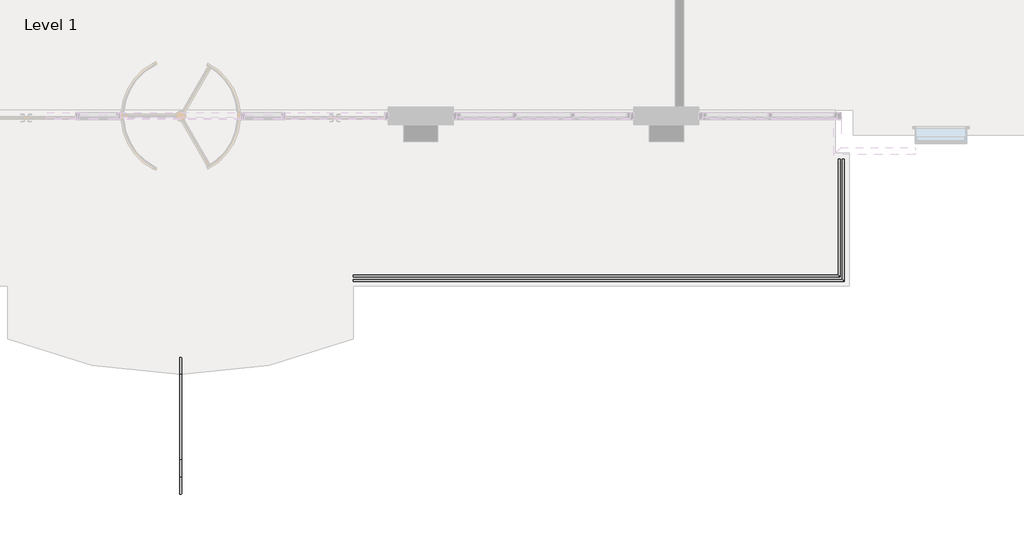
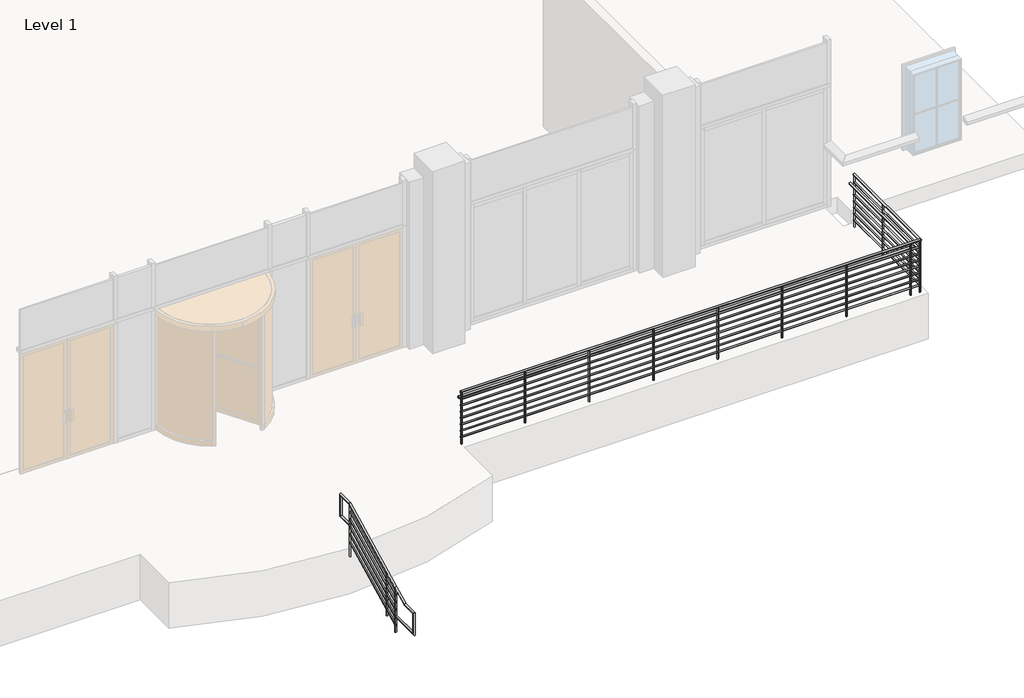
# One storey, part 4 of 6: 2 railings.
"""IFC4 building model written with IfcOpenShell, lengths in millimetres."""

from ifc_helpers import new_model, si_unit, point, frame, frame_2d, origin, origin_with_axes, place, context, project, spatial, circle_curve, ellipse_curve, trimmed, segment, composite_curve, outline, extrude, element, save
from ifc_brep_helpers import plane_surface, cylinder_surface, advanced_brep

model = new_model("IFC4")

# Units and contexts
model_context = context("Model", 3, world=origin())
ifc_project = project(units=[si_unit("LENGTHUNIT", "METRE", prefix="MILLI")], contexts=[model_context])

# Site, building, storey
site = spatial("IfcSite", under=ifc_project)
building = spatial("IfcBuilding", under=site)
storey = spatial("IfcBuildingStorey", under=building, Name="Level 1", Elevation=0.0)

# Railings
placement = place(None, origin())
element("IfcRailing", 1, ObjectType="Handrail – Pipe – Bottom &Top Extension", at=placement, inside=storey, context=model_context, shape_type="AdvancedBrep", body=[
    advanced_brep(
    [(-1146.7622732, -15471.359437, -438.15), (-1184.8622732, -15471.359437, -438.15), (-1146.7622732, -16062.2278525, -438.15), (-1184.8622732, -16062.2278525, -438.15), (-1146.7622732, -16062.2278525, -19.05), (-1184.8622732, -16062.2278525, -19.05), (-1146.7622732, -15771.9807575, -19.05), (-1184.8622732, -15771.9807575, -19.05), (-1146.7622732, -15463.1584335, 135.361162), (-1184.8622732, -15463.1584335, 135.361162), (-1146.7622732, -13943.1807575, 895.35), (-1184.8622732, -13943.1807575, 895.35), (-1146.7622732, -13661.9278525, 895.35), (-1184.8622732, -13661.9278525, 895.35), (-1146.7622732, -13661.9278525, 476.25), (-1184.8622732, -13661.9278525, 476.25), (-1146.7622732, -13947.996268, 476.25), (-1184.8622732, -13947.996268, 476.25)],
    [
        (0, 1, circle_curve(frame((-1165.8122732, -15471.359437, -438.15), z_axis=(0.0, 1.0, 0.0), x_axis=(-1.0, 0.0, 0.0)), 19.05)),
        (1, 0, circle_curve(frame((-1165.8122732, -15471.359437, -438.15), z_axis=(0.0, 1.0, 0.0), x_axis=(-1.0, 0.0, 0.0)), 19.05)),
        (0, 2),
        (2, 3, ellipse_curve(frame((-1165.8122732, -16062.2278525, -438.15), z_axis=(0.0, 0.7071067811865475, -0.7071067811865475), x_axis=(0.0, 0.7071067811865476, 0.7071067811865474)), 26.9407684, 19.05)),
        (3, 1),
        (3, 2, ellipse_curve(frame((-1165.8122732, -16062.2278525, -438.15), z_axis=(0.0, 0.7071067811865475, -0.7071067811865475), x_axis=(0.0, 0.7071067811865476, 0.7071067811865474)), 26.9407684, 19.05)),
        (2, 4),
        (4, 5, ellipse_curve(frame((-1165.8122732, -16062.2278525, -19.05), z_axis=(0.0, -0.7071067811865475, -0.7071067811865475), x_axis=(0.0, 0.7071067811865474, -0.7071067811865476)), 26.9407684, 19.05)),
        (5, 3),
        (5, 4, ellipse_curve(frame((-1165.8122732, -16062.2278525, -19.05), z_axis=(0.0, -0.7071067811865475, -0.7071067811865475), x_axis=(0.0, 0.7071067811865474, -0.7071067811865476)), 26.9407684, 19.05)),
        (4, 6),
        (6, 7, ellipse_curve(frame((-1165.8122732, -15771.9807575, -19.05), z_axis=(0.0, -0.9732489894677302, -0.22975292054736124), x_axis=(0.0, -0.22975292054736096, 0.9732489894677302)), 19.573614, 19.05)),
        (7, 5),
        (7, 6, ellipse_curve(frame((-1165.8122732, -15771.9807575, -19.05), z_axis=(0.0, -0.9732489894677302, -0.22975292054736124), x_axis=(0.0, -0.22975292054736096, 0.9732489894677302)), 19.573614, 19.05)),
        (6, 8),
        (8, 9, circle_curve(frame((-1165.8122732, -15463.1584335, 135.361162), z_axis=(0.0, -0.8944271909999159, -0.44721359549995804), x_axis=(-1.0, 0.0, 0.0)), 19.05)),
        (9, 7),
        (9, 8, circle_curve(frame((-1165.8122732, -15463.1584335, 135.361162), z_axis=(0.0, -0.8944271909999159, -0.44721359549995804), x_axis=(-1.0, 0.0, 0.0)), 19.05)),
        (8, 10),
        (10, 11, ellipse_curve(frame((-1165.8122732, -13943.1807575, 895.35), z_axis=(0.0, -0.9732489894677302, -0.22975292054736132), x_axis=(0.0, 0.2297529205473615, -0.9732489894677301)), 19.573614, 19.05)),
        (11, 9),
        (11, 10, ellipse_curve(frame((-1165.8122732, -13943.1807575, 895.35), z_axis=(0.0, -0.9732489894677302, -0.22975292054736132), x_axis=(0.0, 0.2297529205473615, -0.9732489894677301)), 19.573614, 19.05)),
        (10, 12),
        (12, 13, ellipse_curve(frame((-1165.8122732, -13661.9278525, 895.35), z_axis=(0.0, -0.7071067811865476, 0.7071067811865474), x_axis=(0.0, -0.7071067811865475, -0.7071067811865475)), 26.9407684, 19.05)),
        (13, 11),
        (13, 12, ellipse_curve(frame((-1165.8122732, -13661.9278525, 895.35), z_axis=(0.0, -0.7071067811865476, 0.7071067811865474), x_axis=(0.0, -0.7071067811865475, -0.7071067811865475)), 26.9407684, 19.05)),
        (12, 14),
        (14, 15, ellipse_curve(frame((-1165.8122732, -13661.9278525, 476.25), z_axis=(0.0, 0.7071067811865474, 0.7071067811865476), x_axis=(0.0, -0.7071067811865475, 0.7071067811865475)), 26.9407684, 19.05)),
        (15, 13),
        (15, 14, ellipse_curve(frame((-1165.8122732, -13661.9278525, 476.25), z_axis=(0.0, 0.7071067811865474, 0.7071067811865476), x_axis=(0.0, -0.7071067811865475, 0.7071067811865475)), 26.9407684, 19.05)),
        (16, 17, circle_curve(frame((-1165.8122732, -13947.996268, 476.25), z_axis=(0.0, -1.0, 0.0), x_axis=(-1.0, 0.0, 0.0)), 19.05)),
        (17, 16, circle_curve(frame((-1165.8122732, -13947.996268, 476.25), z_axis=(0.0, -1.0, 0.0), x_axis=(-1.0, 0.0, 0.0)), 19.05)),
        (14, 16),
        (17, 15),
    ],
    [
        plane_surface(frame((-1165.8122732, -15471.359437, -457.2), z_axis=(0.0, 1.0, 0.0), x_axis=(0.0, 0.0, -1.0))),
        cylinder_surface(frame((-1165.8122732, -15471.359437, -438.15), z_axis=(0.0, 1.0, 0.0), x_axis=(-1.0, 0.0, 0.0)), 19.05),
        cylinder_surface(frame((-1165.8122732, -16062.2278525, -457.2), z_axis=(0.0, 0.0, -1.0), x_axis=(-1.0, 0.0, 0.0)), 19.05),
        cylinder_surface(frame((-1165.8122732, -16081.2778525, -19.05), z_axis=(0.0, -1.0, 0.0), x_axis=(-1.0, 0.0, 0.0)), 19.05),
        cylinder_surface(frame((-1165.8122732, -15767.9584335, -17.038838), z_axis=(0.0, -0.8944271909999159, -0.44721359549995804), x_axis=(-1.0, 0.0, 0.0)), 19.05),
        cylinder_surface(frame((-1165.8122732, -15463.1584335, 135.361162), z_axis=(0.0, -0.8944271909999159, -0.44721359549995804), x_axis=(-1.0, 0.0, 0.0)), 19.05),
        cylinder_surface(frame((-1165.8122732, -13947.6778525, 895.35), z_axis=(0.0, -1.0, 0.0), x_axis=(-1.0, 0.0, 0.0)), 19.05),
        cylinder_surface(frame((-1165.8122732, -13661.9278525, 914.4), z_axis=(0.0, 0.0, 1.0), x_axis=(-1.0, 0.0, 0.0)), 19.05),
        plane_surface(frame((-1165.8122732, -13947.996268, 457.2), z_axis=(0.0, -1.0, 0.0), x_axis=(0.0, 0.0, -1.0))),
        cylinder_surface(frame((-1165.8122732, -13642.8778525, 476.25), z_axis=(0.0, 1.0, 0.0), x_axis=(-1.0, 0.0, 0.0)), 19.05),
    ],
    [
        (0, [[1, 2]]),
        (1, [[-1, 3, 4, 5]]),
        (1, [[-2, -5, 6, -3]]),
        (2, [[-4, 7, 8, 9]]),
        (2, [[-6, -9, 10, -7]]),
        (3, [[-8, 11, 12, 13]]),
        (3, [[-10, -13, 14, -11]]),
        (4, [[-12, 15, 16, 17]]),
        (4, [[-14, -17, 18, -15]]),
        (5, [[-16, 19, 20, 21]]),
        (5, [[-18, -21, 22, -19]]),
        (6, [[-20, 23, 24, 25]]),
        (6, [[-22, -25, 26, -23]]),
        (7, [[-24, 27, 28, 29]]),
        (7, [[-26, -29, 30, -27]]),
        (8, [[31, 32]]),
        (9, [[-28, 33, -32, 34]]),
        (9, [[-30, -34, -31, -33]]),
    ],
),
    advanced_brep(
    [(-1153.1122732, -13947.6778525, 747.8009683), (-1178.5122732, -13947.6778525, 747.8009683), (-1153.1122732, -15471.6778525, -14.1990317), (-1178.5122732, -15471.6778525, -14.1990317)],
    [
        (0, 1, ellipse_curve(frame((-1165.8122732, -13947.6778525, 747.8009683), z_axis=(0.0, 1.0, 0.0), x_axis=(0.0, 0.0, 1.0)), 14.1990317, 12.7)),
        (1, 0, ellipse_curve(frame((-1165.8122732, -13947.6778525, 747.8009683), z_axis=(0.0, 1.0, 0.0), x_axis=(0.0, 0.0, 1.0)), 14.1990317, 12.7)),
        (2, 3, ellipse_curve(frame((-1165.8122732, -15471.6778525, -14.1990317), z_axis=(0.0, -1.0, 0.0), x_axis=(0.0, 0.0, 1.0)), 14.1990317, 12.7)),
        (3, 2, ellipse_curve(frame((-1165.8122732, -15471.6778525, -14.1990317), z_axis=(0.0, -1.0, 0.0), x_axis=(0.0, 0.0, 1.0)), 14.1990317, 12.7)),
        (0, 2),
        (3, 1),
    ],
    [
        plane_surface(frame((-1165.8122732, -13947.6778525, 762.0), z_axis=(0.0, 1.0, 0.0), x_axis=(0.0, 0.0, -1.0))),
        plane_surface(frame((-1165.8122732, -15471.6778525, 0.0), z_axis=(0.0, -1.0, 0.0), x_axis=(0.0, 0.0, -1.0))),
        cylinder_surface(frame((-1165.8122732, -13941.9982398, 750.6407747), z_axis=(0.0, 0.894427190999916, 0.447213595499958), x_axis=(-1.0, 0.0, 0.0)), 12.7),
    ],
    [
        (0, [[1, 2]]),
        (1, [[3, 4]]),
        (2, [[-1, 5, -4, 6]]),
        (2, [[-2, -6, -3, -5]]),
    ],
),
    advanced_brep(
    [(-1153.1122732, -13947.6778525, 595.4009683), (-1178.5122732, -13947.6778525, 595.4009683), (-1153.1122732, -15471.6778525, -166.5990317), (-1178.5122732, -15471.6778525, -166.5990317)],
    [
        (0, 1, ellipse_curve(frame((-1165.8122732, -13947.6778525, 595.4009683), z_axis=(0.0, 1.0, 0.0), x_axis=(0.0, 0.0, 1.0)), 14.1990317, 12.7)),
        (1, 0, ellipse_curve(frame((-1165.8122732, -13947.6778525, 595.4009683), z_axis=(0.0, 1.0, 0.0), x_axis=(0.0, 0.0, 1.0)), 14.1990317, 12.7)),
        (2, 3, ellipse_curve(frame((-1165.8122732, -15471.6778525, -166.5990317), z_axis=(0.0, -1.0, 0.0), x_axis=(0.0, 0.0, 1.0)), 14.1990317, 12.7)),
        (3, 2, ellipse_curve(frame((-1165.8122732, -15471.6778525, -166.5990317), z_axis=(0.0, -1.0, 0.0), x_axis=(0.0, 0.0, 1.0)), 14.1990317, 12.7)),
        (0, 2),
        (3, 1),
    ],
    [
        plane_surface(frame((-1165.8122732, -13947.6778525, 609.6), z_axis=(0.0, 1.0, 0.0), x_axis=(0.0, 0.0, -1.0))),
        plane_surface(frame((-1165.8122732, -15471.6778525, -152.4), z_axis=(0.0, -1.0, 0.0), x_axis=(0.0, 0.0, -1.0))),
        cylinder_surface(frame((-1165.8122732, -13941.9982398, 598.2407747), z_axis=(0.0, 0.894427190999916, 0.447213595499958), x_axis=(-1.0, 0.0, 0.0)), 12.7),
    ],
    [
        (0, [[1, 2]]),
        (1, [[3, 4]]),
        (2, [[-1, 5, -4, 6]]),
        (2, [[-2, -6, -3, -5]]),
    ],
),
    advanced_brep(
    [(-1153.1122732, -13947.6778525, 443.0009683), (-1178.5122732, -13947.6778525, 443.0009683), (-1153.1122732, -15471.6778525, -318.9990317), (-1178.5122732, -15471.6778525, -318.9990317)],
    [
        (0, 1, ellipse_curve(frame((-1165.8122732, -13947.6778525, 443.0009683), z_axis=(0.0, 1.0, 0.0), x_axis=(0.0, 0.0, 1.0)), 14.1990317, 12.7)),
        (1, 0, ellipse_curve(frame((-1165.8122732, -13947.6778525, 443.0009683), z_axis=(0.0, 1.0, 0.0), x_axis=(0.0, 0.0, 1.0)), 14.1990317, 12.7)),
        (2, 3, ellipse_curve(frame((-1165.8122732, -15471.6778525, -318.9990317), z_axis=(0.0, -1.0, 0.0), x_axis=(0.0, 0.0, 1.0)), 14.1990317, 12.7)),
        (3, 2, ellipse_curve(frame((-1165.8122732, -15471.6778525, -318.9990317), z_axis=(0.0, -1.0, 0.0), x_axis=(0.0, 0.0, 1.0)), 14.1990317, 12.7)),
        (0, 2),
        (3, 1),
    ],
    [
        plane_surface(frame((-1165.8122732, -13947.6778525, 457.2), z_axis=(0.0, 1.0, 0.0), x_axis=(0.0, 0.0, -1.0))),
        plane_surface(frame((-1165.8122732, -15471.6778525, -304.8), z_axis=(0.0, -1.0, 0.0), x_axis=(0.0, 0.0, -1.0))),
        cylinder_surface(frame((-1165.8122732, -13941.9982398, 445.8407747), z_axis=(0.0, 0.894427190999916, 0.447213595499958), x_axis=(-1.0, 0.0, 0.0)), 12.7),
    ],
    [
        (0, [[1, 2]]),
        (1, [[3, 4]]),
        (2, [[-1, 5, -4, 6]]),
        (2, [[-2, -6, -3, -5]]),
    ],
),
    advanced_brep(
    [(-1153.1122732, -13947.6778525, 290.6009683), (-1178.5122732, -13947.6778525, 290.6009683), (-1153.1122732, -15471.6778525, -471.3990317), (-1178.5122732, -15471.6778525, -471.3990317)],
    [
        (0, 1, ellipse_curve(frame((-1165.8122732, -13947.6778525, 290.6009683), z_axis=(0.0, 1.0, 0.0), x_axis=(0.0, 0.0, 1.0)), 14.1990317, 12.7)),
        (1, 0, ellipse_curve(frame((-1165.8122732, -13947.6778525, 290.6009683), z_axis=(0.0, 1.0, 0.0), x_axis=(0.0, 0.0, 1.0)), 14.1990317, 12.7)),
        (2, 3, ellipse_curve(frame((-1165.8122732, -15471.6778525, -471.3990317), z_axis=(0.0, -1.0, 0.0), x_axis=(0.0, 0.0, 1.0)), 14.1990317, 12.7)),
        (3, 2, ellipse_curve(frame((-1165.8122732, -15471.6778525, -471.3990317), z_axis=(0.0, -1.0, 0.0), x_axis=(0.0, 0.0, 1.0)), 14.1990317, 12.7)),
        (0, 2),
        (3, 1),
    ],
    [
        plane_surface(frame((-1165.8122732, -13947.6778525, 304.8), z_axis=(0.0, 1.0, 0.0), x_axis=(0.0, 0.0, -1.0))),
        plane_surface(frame((-1165.8122732, -15471.6778525, -457.2), z_axis=(0.0, -1.0, 0.0), x_axis=(0.0, 0.0, -1.0))),
        cylinder_surface(frame((-1165.8122732, -13941.9982398, 293.4407747), z_axis=(0.0, 0.894427190999916, 0.447213595499958), x_axis=(-1.0, 0.0, 0.0)), 12.7),
    ],
    [
        (0, [[1, 2]]),
        (1, [[3, 4]]),
        (2, [[-1, 5, -4, 6]]),
        (2, [[-2, -6, -3, -5]]),
    ],
),
    advanced_brep(
    [(-1153.1122732, -13947.6778525, 138.2009683), (-1178.5122732, -13947.6778525, 138.2009683), (-1153.1122732, -15471.6778525, -623.7990317), (-1178.5122732, -15471.6778525, -623.7990317)],
    [
        (0, 1, ellipse_curve(frame((-1165.8122732, -13947.6778525, 138.2009683), z_axis=(0.0, 1.0, 0.0), x_axis=(0.0, 0.0, 1.0)), 14.1990317, 12.7)),
        (1, 0, ellipse_curve(frame((-1165.8122732, -13947.6778525, 138.2009683), z_axis=(0.0, 1.0, 0.0), x_axis=(0.0, 0.0, 1.0)), 14.1990317, 12.7)),
        (2, 3, ellipse_curve(frame((-1165.8122732, -15471.6778525, -623.7990317), z_axis=(0.0, -1.0, 0.0), x_axis=(0.0, 0.0, 1.0)), 14.1990317, 12.7)),
        (3, 2, ellipse_curve(frame((-1165.8122732, -15471.6778525, -623.7990317), z_axis=(0.0, -1.0, 0.0), x_axis=(0.0, 0.0, 1.0)), 14.1990317, 12.7)),
        (0, 2),
        (3, 1),
    ],
    [
        plane_surface(frame((-1165.8122732, -13947.6778525, 152.4), z_axis=(0.0, 1.0, 0.0), x_axis=(0.0, 0.0, -1.0))),
        plane_surface(frame((-1165.8122732, -15471.6778525, -609.6), z_axis=(0.0, -1.0, 0.0), x_axis=(0.0, 0.0, -1.0))),
        cylinder_surface(frame((-1165.8122732, -13941.9982398, 141.0407747), z_axis=(0.0, 0.894427190999916, 0.447213595499958), x_axis=(-1.0, 0.0, 0.0)), 12.7),
    ],
    [
        (0, [[1, 2]]),
        (1, [[3, 4]]),
        (2, [[-1, 5, -4, 6]]),
        (2, [[-2, -6, -3, -5]]),
    ],
),
    advanced_brep(
    [(-1178.5122732, -15166.8778525, 262.202905), (-1178.5122732, -15166.8778525, -609.6), (-1153.1122732, -15166.8778525, -609.6), (-1153.1122732, -15166.8778525, 262.202905)],
    [
        (0, 1),
        (1, 2, circle_curve(frame((-1165.8122732, -15166.8778525, -609.6), z_axis=(0.0, 0.0, 1.0), x_axis=(1.0, 0.0, 0.0)), 12.7)),
        (2, 3),
        (3, 0, ellipse_curve(frame((-1165.8122732, -15166.8778525, 262.202905), z_axis=(0.0, 0.4472135954999566, -0.8944271909999165), x_axis=(0.0, 0.8944271909999165, 0.4472135954999567)), 14.1990317, 12.7)),
        (0, 3, ellipse_curve(frame((-1165.8122732, -15166.8778525, 262.202905), z_axis=(0.0, 0.4472135954999566, -0.8944271909999165), x_axis=(0.0, 0.8944271909999165, 0.4472135954999567)), 14.1990317, 12.7)),
        (2, 1, circle_curve(frame((-1165.8122732, -15166.8778525, -609.6), z_axis=(0.0, 0.0, 1.0), x_axis=(1.0, 0.0, 0.0)), 12.7)),
    ],
    [
        cylinder_surface(frame((-1165.8122732, -15166.8778525, -838.2), z_axis=(0.0, 0.0, 1.0), x_axis=(1.0, 0.0, 0.0)), 12.7),
        plane_surface(frame((-1140.4122732, -15192.2778525, 249.502905), z_axis=(0.0, -0.4472135954999566, 0.8944271909999165), x_axis=(-1.0, 0.0, 0.0))),
        plane_surface(frame((-1140.4122732, -15141.4778525, -609.6), z_axis=(0.0, 0.0, -1.0), x_axis=(-1.0, 0.0, 0.0))),
    ],
    [
        (0, [[1, 2, 3, 4]]),
        (0, [[-1, 5, -3, 6]]),
        (1, [[-4, -5]]),
        (2, [[-2, -6]]),
    ],
),
    advanced_brep(
    [(-1178.5122732, -15458.9778525, 116.152905), (-1178.5122732, -15458.9778525, -762.0), (-1153.1122732, -15458.9778525, -762.0), (-1153.1122732, -15458.9778525, 116.152905)],
    [
        (0, 1),
        (1, 2, circle_curve(frame((-1165.8122732, -15458.9778525, -762.0), z_axis=(0.0, 0.0, 1.0), x_axis=(1.0, 0.0, 0.0)), 12.7)),
        (2, 3),
        (3, 0, ellipse_curve(frame((-1165.8122732, -15458.9778525, 116.152905), z_axis=(0.0, 0.4472135954999566, -0.8944271909999165), x_axis=(0.0, 0.8944271909999165, 0.4472135954999567)), 14.1990317, 12.7)),
        (0, 3, ellipse_curve(frame((-1165.8122732, -15458.9778525, 116.152905), z_axis=(0.0, 0.4472135954999566, -0.8944271909999165), x_axis=(0.0, 0.8944271909999165, 0.4472135954999567)), 14.1990317, 12.7)),
        (2, 1, circle_curve(frame((-1165.8122732, -15458.9778525, -762.0), z_axis=(0.0, 0.0, 1.0), x_axis=(1.0, 0.0, 0.0)), 12.7)),
    ],
    [
        cylinder_surface(frame((-1165.8122732, -15458.9778525, -990.6), z_axis=(0.0, 0.0, 1.0), x_axis=(1.0, 0.0, 0.0)), 12.7),
        plane_surface(frame((-1140.4122732, -15484.3778525, 103.452905), z_axis=(0.0, -0.4472135954999566, 0.8944271909999165), x_axis=(-1.0, 0.0, 0.0))),
        plane_surface(frame((-1140.4122732, -15433.5778525, -762.0), z_axis=(0.0, 0.0, -1.0), x_axis=(-1.0, 0.0, 0.0))),
    ],
    [
        (0, [[1, 2, 3, 4]]),
        (0, [[-1, 5, -3, 6]]),
        (1, [[-4, -5]]),
        (2, [[-2, -6]]),
    ],
),
    advanced_brep(
    [(-1178.5122732, -13960.3778525, 865.452905), (-1178.5122732, -13960.3778525, -152.4), (-1153.1122732, -13960.3778525, -152.4), (-1153.1122732, -13960.3778525, 865.452905)],
    [
        (0, 1),
        (1, 2, circle_curve(frame((-1165.8122732, -13960.3778525, -152.4), z_axis=(0.0, 0.0, 1.0), x_axis=(1.0, 0.0, 0.0)), 12.7)),
        (2, 3),
        (3, 0, ellipse_curve(frame((-1165.8122732, -13960.3778525, 865.452905), z_axis=(0.0, 0.4472135954999566, -0.8944271909999165), x_axis=(0.0, 0.8944271909999165, 0.4472135954999567)), 14.1990317, 12.7)),
        (0, 3, ellipse_curve(frame((-1165.8122732, -13960.3778525, 865.452905), z_axis=(0.0, 0.4472135954999566, -0.8944271909999165), x_axis=(0.0, 0.8944271909999165, 0.4472135954999567)), 14.1990317, 12.7)),
        (2, 1, circle_curve(frame((-1165.8122732, -13960.3778525, -152.4), z_axis=(0.0, 0.0, 1.0), x_axis=(1.0, 0.0, 0.0)), 12.7)),
    ],
    [
        cylinder_surface(frame((-1165.8122732, -13960.3778525, -381.0), z_axis=(0.0, 0.0, 1.0), x_axis=(1.0, 0.0, 0.0)), 12.7),
        plane_surface(frame((-1140.4122732, -13985.7778525, 852.752905), z_axis=(0.0, -0.4472135954999566, 0.8944271909999165), x_axis=(-1.0, 0.0, 0.0))),
        plane_surface(frame((-1140.4122732, -13934.9778525, -152.4), z_axis=(0.0, 0.0, -1.0), x_axis=(-1.0, 0.0, 0.0))),
    ],
    [
        (0, [[1, 2, 3, 4]]),
        (0, [[-1, 5, -3, 6]]),
        (1, [[-4, -5]]),
        (2, [[-2, -6]]),
    ],
),
])
element("IfcRailing", 2, ObjectType="Guardrail - Pipe", at=placement, inside=storey, context=model_context, shape_type="SolidModel", body=[
    advanced_brep(
    [(1903.9547354, -12217.7608439, 895.35), (1903.9547354, -12179.6608439, 895.35), (10558.224655, -12217.7608439, 895.35), (10520.124655, -12179.6608439, 895.35), (10558.224655, -10114.0984696, 895.35), (10520.124655, -10114.0984696, 895.35)],
    [
        (0, 1, circle_curve(frame((1903.9547354, -12198.7108439, 895.35), z_axis=(-1.0, 0.0, 0.0), x_axis=(0.0, 1.0, 0.0)), 19.05)),
        (1, 0, circle_curve(frame((1903.9547354, -12198.7108439, 895.35), z_axis=(-1.0, 0.0, 0.0), x_axis=(0.0, 1.0, 0.0)), 19.05)),
        (0, 2),
        (2, 3, ellipse_curve(frame((10539.174655, -12198.7108439, 895.35), z_axis=(-0.7071067811865475, -0.7071067811865475, 0.0), x_axis=(-0.7071067811865476, 0.7071067811865474, 0.0)), 26.9407684, 19.05)),
        (3, 1),
        (3, 2, ellipse_curve(frame((10539.174655, -12198.7108439, 895.35), z_axis=(-0.7071067811865475, -0.7071067811865475, 0.0), x_axis=(-0.7071067811865476, 0.7071067811865474, 0.0)), 26.9407684, 19.05)),
        (4, 5, circle_curve(frame((10539.174655, -10114.0984696, 895.35), z_axis=(0.0, 1.0, 0.0), x_axis=(-1.0, 0.0, 0.0)), 19.05)),
        (5, 4, circle_curve(frame((10539.174655, -10114.0984696, 895.35), z_axis=(0.0, 1.0, 0.0), x_axis=(-1.0, 0.0, 0.0)), 19.05)),
        (2, 4),
        (5, 3),
    ],
    [
        plane_surface(frame((1903.9547354, -12198.7108439, 914.4), z_axis=(-1.0, 0.0, 0.0), x_axis=(0.0, 1.0, 0.0))),
        cylinder_surface(frame((1903.9547354, -12198.7108439, 895.35), z_axis=(-1.0, 0.0, 0.0), x_axis=(0.0, 1.0, 0.0)), 19.05),
        plane_surface(frame((10539.174655, -10114.0984696, 914.4), z_axis=(0.0, 1.0, 0.0), x_axis=(0.0, 0.0, 1.0))),
        cylinder_surface(frame((10539.174655, -12198.7108439, 895.35), z_axis=(0.0, -1.0, 0.0), x_axis=(-1.0, 0.0, 0.0)), 19.05),
    ],
    [
        (0, [[1, 2]]),
        (1, [[-1, 3, 4, 5]]),
        (1, [[-2, -5, 6, -3]]),
        (2, [[7, 8]]),
        (3, [[-4, 9, -8, 10]]),
        (3, [[-6, -10, -7, -9]]),
    ],
),
    advanced_brep(
    [(1903.9547354, -12293.9608439, 1047.75), (1903.9547354, -12255.8608439, 1047.75), (10634.424655, -12293.9608439, 1047.75), (10596.324655, -12255.8608439, 1047.75), (10634.424655, -10114.0984696, 1047.75), (10596.324655, -10114.0984696, 1047.75)],
    [
        (0, 1, circle_curve(frame((1903.9547354, -12274.9108439, 1047.75), z_axis=(-1.0, 0.0, 0.0), x_axis=(0.0, 1.0, 0.0)), 19.05)),
        (1, 0, circle_curve(frame((1903.9547354, -12274.9108439, 1047.75), z_axis=(-1.0, 0.0, 0.0), x_axis=(0.0, 1.0, 0.0)), 19.05)),
        (0, 2),
        (2, 3, ellipse_curve(frame((10615.374655, -12274.9108439, 1047.75), z_axis=(-0.7071067811865475, -0.7071067811865475, 0.0), x_axis=(-0.7071067811865476, 0.7071067811865474, 0.0)), 26.9407684, 19.05)),
        (3, 1),
        (3, 2, ellipse_curve(frame((10615.374655, -12274.9108439, 1047.75), z_axis=(-0.7071067811865475, -0.7071067811865475, 0.0), x_axis=(-0.7071067811865476, 0.7071067811865474, 0.0)), 26.9407684, 19.05)),
        (4, 5, circle_curve(frame((10615.374655, -10114.0984696, 1047.75), z_axis=(0.0, 1.0, 0.0), x_axis=(-1.0, 0.0, 0.0)), 19.05)),
        (5, 4, circle_curve(frame((10615.374655, -10114.0984696, 1047.75), z_axis=(0.0, 1.0, 0.0), x_axis=(-1.0, 0.0, 0.0)), 19.05)),
        (2, 4),
        (5, 3),
    ],
    [
        plane_surface(frame((1903.9547354, -12274.9108439, 1066.8), z_axis=(-1.0, 0.0, 0.0), x_axis=(0.0, 1.0, 0.0))),
        cylinder_surface(frame((1903.9547354, -12274.9108439, 1047.75), z_axis=(-1.0, 0.0, 0.0), x_axis=(0.0, 1.0, 0.0)), 19.05),
        plane_surface(frame((10615.374655, -10114.0984696, 1066.8), z_axis=(0.0, 1.0, 0.0), x_axis=(0.0, 0.0, 1.0))),
        cylinder_surface(frame((10615.374655, -12274.9108439, 1047.75), z_axis=(0.0, -1.0, 0.0), x_axis=(-1.0, 0.0, 0.0)), 19.05),
    ],
    [
        (0, [[1, 2]]),
        (1, [[-1, 3, 4, 5]]),
        (1, [[-2, -5, 6, -3]]),
        (2, [[7, 8]]),
        (3, [[-4, 9, -8, 10]]),
        (3, [[-6, -10, -7, -9]]),
    ],
),
    extrude(outline(composite_curve([segment(trimmed(circle_curve(frame_2d((-12274.9108439, 901.7)), 12.7), [point((-12262.2108439, 901.7))], [point((-12287.6108439, 901.7))], False, "CARTESIAN"), True, "CONTINUOUS"), segment(trimmed(circle_curve(frame_2d((-12274.9108439, 901.7)), 12.7), [point((-12287.6108439, 901.7))], [point((-12262.2108439, 901.7))], False, "CARTESIAN"), True, "CONTINUOUS")], self_intersect=False)), frame((1903.9547354, 0.0, 0.0), z_axis=(1.0, 0.0, 0.0), x_axis=(0.0, 1.0, 0.0)), (0.0, 0.0, 1.0), 8698.7199196),
    extrude(outline(composite_curve([segment(trimmed(circle_curve(frame_2d((901.7, 10615.374655)), 12.7), [point((901.7, 10602.674655))], [point((901.7, 10628.074655))], False, "CARTESIAN"), True, "CONTINUOUS"), segment(trimmed(circle_curve(frame_2d((901.7, 10615.374655)), 12.7), [point((901.7, 10628.074655))], [point((901.7, 10602.674655))], False, "CARTESIAN"), True, "CONTINUOUS")], self_intersect=False)), frame((0.0, -12287.6108439, 0.0), z_axis=(0.0, 1.0, 0.0), x_axis=(0.0, 0.0, 1.0)), (0.0, 0.0, 1.0), 2173.5123743),
    extrude(outline(composite_curve([segment(trimmed(circle_curve(frame_2d((-12274.9108439, 774.7)), 12.7), [point((-12262.2108439, 774.7))], [point((-12287.6108439, 774.7))], False, "CARTESIAN"), True, "CONTINUOUS"), segment(trimmed(circle_curve(frame_2d((-12274.9108439, 774.7)), 12.7), [point((-12287.6108439, 774.7))], [point((-12262.2108439, 774.7))], False, "CARTESIAN"), True, "CONTINUOUS")], self_intersect=False)), frame((1903.9547354, 0.0, 0.0), z_axis=(1.0, 0.0, 0.0), x_axis=(0.0, 1.0, 0.0)), (0.0, 0.0, 1.0), 8698.7199196),
    extrude(outline(composite_curve([segment(trimmed(circle_curve(frame_2d((774.7, 10615.374655)), 12.7), [point((774.7, 10602.674655))], [point((774.7, 10628.074655))], False, "CARTESIAN"), True, "CONTINUOUS"), segment(trimmed(circle_curve(frame_2d((774.7, 10615.374655)), 12.7), [point((774.7, 10628.074655))], [point((774.7, 10602.674655))], False, "CARTESIAN"), True, "CONTINUOUS")], self_intersect=False)), frame((0.0, -12287.6108439, 0.0), z_axis=(0.0, 1.0, 0.0), x_axis=(0.0, 0.0, 1.0)), (0.0, 0.0, 1.0), 2173.5123743),
    extrude(outline(composite_curve([segment(trimmed(circle_curve(frame_2d((-12274.9108439, 647.7)), 12.7), [point((-12262.2108439, 647.7))], [point((-12287.6108439, 647.7))], False, "CARTESIAN"), True, "CONTINUOUS"), segment(trimmed(circle_curve(frame_2d((-12274.9108439, 647.7)), 12.7), [point((-12287.6108439, 647.7))], [point((-12262.2108439, 647.7))], False, "CARTESIAN"), True, "CONTINUOUS")], self_intersect=False)), frame((1903.9547354, 0.0, 0.0), z_axis=(1.0, 0.0, 0.0), x_axis=(0.0, 1.0, 0.0)), (0.0, 0.0, 1.0), 8698.7199196),
    extrude(outline(composite_curve([segment(trimmed(circle_curve(frame_2d((647.7, 10615.374655)), 12.7), [point((647.7, 10602.674655))], [point((647.7, 10628.074655))], False, "CARTESIAN"), True, "CONTINUOUS"), segment(trimmed(circle_curve(frame_2d((647.7, 10615.374655)), 12.7), [point((647.7, 10628.074655))], [point((647.7, 10602.674655))], False, "CARTESIAN"), True, "CONTINUOUS")], self_intersect=False)), frame((0.0, -12287.6108439, 0.0), z_axis=(0.0, 1.0, 0.0), x_axis=(0.0, 0.0, 1.0)), (0.0, 0.0, 1.0), 2173.5123743),
    extrude(outline(composite_curve([segment(trimmed(circle_curve(frame_2d((-12274.9108439, 520.7)), 12.7), [point((-12262.2108439, 520.7))], [point((-12287.6108439, 520.7))], False, "CARTESIAN"), True, "CONTINUOUS"), segment(trimmed(circle_curve(frame_2d((-12274.9108439, 520.7)), 12.7), [point((-12287.6108439, 520.7))], [point((-12262.2108439, 520.7))], False, "CARTESIAN"), True, "CONTINUOUS")], self_intersect=False)), frame((1903.9547354, 0.0, 0.0), z_axis=(1.0, 0.0, 0.0), x_axis=(0.0, 1.0, 0.0)), (0.0, 0.0, 1.0), 8698.7199196),
    extrude(outline(composite_curve([segment(trimmed(circle_curve(frame_2d((520.7, 10615.374655)), 12.7), [point((520.7, 10602.674655))], [point((520.7, 10628.074655))], False, "CARTESIAN"), True, "CONTINUOUS"), segment(trimmed(circle_curve(frame_2d((520.7, 10615.374655)), 12.7), [point((520.7, 10628.074655))], [point((520.7, 10602.674655))], False, "CARTESIAN"), True, "CONTINUOUS")], self_intersect=False)), frame((0.0, -12287.6108439, 0.0), z_axis=(0.0, 1.0, 0.0), x_axis=(0.0, 0.0, 1.0)), (0.0, 0.0, 1.0), 2173.5123743),
    extrude(outline(composite_curve([segment(trimmed(circle_curve(frame_2d((-12274.9108439, 393.7)), 12.7), [point((-12262.2108439, 393.7))], [point((-12287.6108439, 393.7))], False, "CARTESIAN"), True, "CONTINUOUS"), segment(trimmed(circle_curve(frame_2d((-12274.9108439, 393.7)), 12.7), [point((-12287.6108439, 393.7))], [point((-12262.2108439, 393.7))], False, "CARTESIAN"), True, "CONTINUOUS")], self_intersect=False)), frame((1903.9547354, 0.0, 0.0), z_axis=(1.0, 0.0, 0.0), x_axis=(0.0, 1.0, 0.0)), (0.0, 0.0, 1.0), 8698.7199196),
    extrude(outline(composite_curve([segment(trimmed(circle_curve(frame_2d((393.7, 10615.374655)), 12.7), [point((393.7, 10602.674655))], [point((393.7, 10628.074655))], False, "CARTESIAN"), True, "CONTINUOUS"), segment(trimmed(circle_curve(frame_2d((393.7, 10615.374655)), 12.7), [point((393.7, 10628.074655))], [point((393.7, 10602.674655))], False, "CARTESIAN"), True, "CONTINUOUS")], self_intersect=False)), frame((0.0, -12287.6108439, 0.0), z_axis=(0.0, 1.0, 0.0), x_axis=(0.0, 0.0, 1.0)), (0.0, 0.0, 1.0), 2173.5123743),
    extrude(outline(composite_curve([segment(trimmed(circle_curve(frame_2d((-12274.9108439, 266.7)), 12.7), [point((-12262.2108439, 266.7))], [point((-12287.6108439, 266.7))], False, "CARTESIAN"), True, "CONTINUOUS"), segment(trimmed(circle_curve(frame_2d((-12274.9108439, 266.7)), 12.7), [point((-12287.6108439, 266.7))], [point((-12262.2108439, 266.7))], False, "CARTESIAN"), True, "CONTINUOUS")], self_intersect=False)), frame((1903.9547354, 0.0, 0.0), z_axis=(1.0, 0.0, 0.0), x_axis=(0.0, 1.0, 0.0)), (0.0, 0.0, 1.0), 8698.7199196),
    extrude(outline(composite_curve([segment(trimmed(circle_curve(frame_2d((266.7, 10615.374655)), 12.7), [point((266.7, 10602.674655))], [point((266.7, 10628.074655))], False, "CARTESIAN"), True, "CONTINUOUS"), segment(trimmed(circle_curve(frame_2d((266.7, 10615.374655)), 12.7), [point((266.7, 10628.074655))], [point((266.7, 10602.674655))], False, "CARTESIAN"), True, "CONTINUOUS")], self_intersect=False)), frame((0.0, -12287.6108439, 0.0), z_axis=(0.0, 1.0, 0.0), x_axis=(0.0, 0.0, 1.0)), (0.0, 0.0, 1.0), 2173.5123743),
    extrude(outline(composite_curve([segment(trimmed(circle_curve(frame_2d((-12274.9108439, 139.7)), 12.7), [point((-12262.2108439, 139.7))], [point((-12287.6108439, 139.7))], False, "CARTESIAN"), True, "CONTINUOUS"), segment(trimmed(circle_curve(frame_2d((-12274.9108439, 139.7)), 12.7), [point((-12287.6108439, 139.7))], [point((-12262.2108439, 139.7))], False, "CARTESIAN"), True, "CONTINUOUS")], self_intersect=False)), frame((1903.9547354, 0.0, 0.0), z_axis=(1.0, 0.0, 0.0), x_axis=(0.0, 1.0, 0.0)), (0.0, 0.0, 1.0), 8698.7199196),
    extrude(outline(composite_curve([segment(trimmed(circle_curve(frame_2d((139.7, 10615.374655)), 12.7), [point((139.7, 10602.674655))], [point((139.7, 10628.074655))], False, "CARTESIAN"), True, "CONTINUOUS"), segment(trimmed(circle_curve(frame_2d((139.7, 10615.374655)), 12.7), [point((139.7, 10628.074655))], [point((139.7, 10602.674655))], False, "CARTESIAN"), True, "CONTINUOUS")], self_intersect=False)), frame((0.0, -12287.6108439, 0.0), z_axis=(0.0, 1.0, 0.0), x_axis=(0.0, 0.0, 1.0)), (0.0, 0.0, 1.0), 2173.5123743),
    extrude(outline(composite_curve([segment(trimmed(circle_curve(frame_2d((10615.374655, -11055.7108439)), 12.7), [point((10602.674655, -11055.7108439))], [point((10628.074655, -11055.7108439))], False, "CARTESIAN"), True, "CONTINUOUS"), segment(trimmed(circle_curve(frame_2d((10615.374655, -11055.7108439)), 12.7), [point((10628.074655, -11055.7108439))], [point((10602.674655, -11055.7108439))], False, "CARTESIAN"), True, "CONTINUOUS")], self_intersect=False)), origin_with_axes(), (0.0, 0.0, 1.0), 1028.7),
    extrude(outline(composite_curve([segment(trimmed(circle_curve(frame_2d((10438.3547354, -12274.9108439)), 12.7), [point((10438.3547354, -12262.2108439))], [point((10438.3547354, -12287.6108439))], False, "CARTESIAN"), True, "CONTINUOUS"), segment(trimmed(circle_curve(frame_2d((10438.3547354, -12274.9108439)), 12.7), [point((10438.3547354, -12287.6108439))], [point((10438.3547354, -12262.2108439))], False, "CARTESIAN"), True, "CONTINUOUS")], self_intersect=False)), origin_with_axes(), (0.0, 0.0, 1.0), 1028.7),
    extrude(outline(composite_curve([segment(trimmed(circle_curve(frame_2d((9219.1547354, -12274.9108439)), 12.7), [point((9219.1547354, -12262.2108439))], [point((9219.1547354, -12287.6108439))], False, "CARTESIAN"), True, "CONTINUOUS"), segment(trimmed(circle_curve(frame_2d((9219.1547354, -12274.9108439)), 12.7), [point((9219.1547354, -12287.6108439))], [point((9219.1547354, -12262.2108439))], False, "CARTESIAN"), True, "CONTINUOUS")], self_intersect=False)), origin_with_axes(), (0.0, 0.0, 1.0), 1028.7),
    extrude(outline(composite_curve([segment(trimmed(circle_curve(frame_2d((7999.9547354, -12274.9108439)), 12.7), [point((7999.9547354, -12262.2108439))], [point((7999.9547354, -12287.6108439))], False, "CARTESIAN"), True, "CONTINUOUS"), segment(trimmed(circle_curve(frame_2d((7999.9547354, -12274.9108439)), 12.7), [point((7999.9547354, -12287.6108439))], [point((7999.9547354, -12262.2108439))], False, "CARTESIAN"), True, "CONTINUOUS")], self_intersect=False)), origin_with_axes(), (0.0, 0.0, 1.0), 1028.7),
    extrude(outline(composite_curve([segment(trimmed(circle_curve(frame_2d((6780.7547354, -12274.9108439)), 12.7), [point((6780.7547354, -12262.2108439))], [point((6780.7547354, -12287.6108439))], False, "CARTESIAN"), True, "CONTINUOUS"), segment(trimmed(circle_curve(frame_2d((6780.7547354, -12274.9108439)), 12.7), [point((6780.7547354, -12287.6108439))], [point((6780.7547354, -12262.2108439))], False, "CARTESIAN"), True, "CONTINUOUS")], self_intersect=False)), origin_with_axes(), (0.0, 0.0, 1.0), 1028.7),
    extrude(outline(composite_curve([segment(trimmed(circle_curve(frame_2d((5561.5547354, -12274.9108439)), 12.7), [point((5561.5547354, -12262.2108439))], [point((5561.5547354, -12287.6108439))], False, "CARTESIAN"), True, "CONTINUOUS"), segment(trimmed(circle_curve(frame_2d((5561.5547354, -12274.9108439)), 12.7), [point((5561.5547354, -12287.6108439))], [point((5561.5547354, -12262.2108439))], False, "CARTESIAN"), True, "CONTINUOUS")], self_intersect=False)), origin_with_axes(), (0.0, 0.0, 1.0), 1028.7),
    extrude(outline(composite_curve([segment(trimmed(circle_curve(frame_2d((4342.3547354, -12274.9108439)), 12.7), [point((4342.3547354, -12262.2108439))], [point((4342.3547354, -12287.6108439))], False, "CARTESIAN"), True, "CONTINUOUS"), segment(trimmed(circle_curve(frame_2d((4342.3547354, -12274.9108439)), 12.7), [point((4342.3547354, -12287.6108439))], [point((4342.3547354, -12262.2108439))], False, "CARTESIAN"), True, "CONTINUOUS")], self_intersect=False)), origin_with_axes(), (0.0, 0.0, 1.0), 1028.7),
    extrude(outline(composite_curve([segment(trimmed(circle_curve(frame_2d((3123.1547354, -12274.9108439)), 12.7), [point((3123.1547354, -12262.2108439))], [point((3123.1547354, -12287.6108439))], False, "CARTESIAN"), True, "CONTINUOUS"), segment(trimmed(circle_curve(frame_2d((3123.1547354, -12274.9108439)), 12.7), [point((3123.1547354, -12287.6108439))], [point((3123.1547354, -12262.2108439))], False, "CARTESIAN"), True, "CONTINUOUS")], self_intersect=False)), origin_with_axes(), (0.0, 0.0, 1.0), 1028.7),
    extrude(outline(composite_curve([segment(trimmed(circle_curve(frame_2d((10615.374655, -12274.9108439)), 12.7), [point((10615.374655, -12262.2108439))], [point((10615.374655, -12287.6108439))], False, "CARTESIAN"), True, "CONTINUOUS"), segment(trimmed(circle_curve(frame_2d((10615.374655, -12274.9108439)), 12.7), [point((10615.374655, -12287.6108439))], [point((10615.374655, -12262.2108439))], False, "CARTESIAN"), True, "CONTINUOUS")], self_intersect=False)), origin_with_axes(), (0.0, 0.0, 1.0), 1028.7),
    extrude(outline(composite_curve([segment(trimmed(circle_curve(frame_2d((10615.374655, -10126.7984696)), 12.7), [point((10602.674655, -10126.7984696))], [point((10628.074655, -10126.7984696))], False, "CARTESIAN"), True, "CONTINUOUS"), segment(trimmed(circle_curve(frame_2d((10615.374655, -10126.7984696)), 12.7), [point((10628.074655, -10126.7984696))], [point((10602.674655, -10126.7984696))], False, "CARTESIAN"), True, "CONTINUOUS")], self_intersect=False)), origin_with_axes(), (0.0, 0.0, 1.0), 1028.7),
    extrude(outline(composite_curve([segment(trimmed(circle_curve(frame_2d((1916.6547354, -12274.9108439)), 12.7), [point((1916.6547354, -12262.2108439))], [point((1916.6547354, -12287.6108439))], False, "CARTESIAN"), True, "CONTINUOUS"), segment(trimmed(circle_curve(frame_2d((1916.6547354, -12274.9108439)), 12.7), [point((1916.6547354, -12287.6108439))], [point((1916.6547354, -12262.2108439))], False, "CARTESIAN"), True, "CONTINUOUS")], self_intersect=False)), origin_with_axes(), (0.0, 0.0, 1.0), 1028.7),
])

save(model, "model.ifc")

# Revit data of these elements
# Project information
#   Organization Name = "G3B Press"
#   Organization Description = "Paul F. Aubin Cosulting Services, Inc."
#   Building Name = "Revit Essentials for Architecture"
#   Author = "Paul F. Aubin"
#   Author Website = "https://www.paulaubin.com"
#   Copyright = "Copyright © 2020 Paul F Aubin, all rights reserved"
#   Design Option = "Main Model"
#   Project Issue Date = "8/1/2020"
#   Project Status = "Design Development"
#   Client Name = "Ceiling Plans and Interior Elevations"
#   Project Address = "123 State ST\nSuite 301\nChicago, IL 60606"
#   Project Name = "14 Commercial_Complete"
#   Project Number = "2020.04A"
# Grids (mm)
#   "1": line (-22547.601, -9504.498) -> (19277.595, -9504.498)
#   "2": line (-22547.601, -3408.498) -> (19277.595, -3408.498)
#   "3": line (-22547.601, 3093.902) -> (19277.595, 3093.902)
#   "4": line (-22547.601, 9189.902) -> (19277.595, 9189.902)
#   "A": line (-16558.212, 12259.726) -> (-16558.212, -14197.104)
#   "B": line (-9801.812, 12259.726) -> (-9801.812, -14197.104)
#   "C": line (-5433.012, 12259.726) -> (-5433.012, -14197.104)
#   "D": line (3101.388, 12259.726) -> (3101.388, -14197.104)
#   "E": line (7470.188, 12259.726) -> (7470.188, -14197.104)
#   "F": line (14226.588, 12259.726) -> (14226.588, -14197.104)
#   "C.3": line (-2689.812, -15151.11) -> (-2689.812, -5965.346)
#   "C.7": line (358.188, -15151.11) -> (358.188, -5965.346)
# Type "Handrail – Pipe – Bottom &Top Extension"
#   Assembly Code = "C2010400"
#   built-in parameter 1008612 = 0.0416667 (stored number, unit not read)
#   built-in parameter 1008611 = 0.0833333 (stored number, unit not read)
#   built-in parameter 1008609 = 4 (stored number, unit not read)
#   built-in parameter 1008604 = 0.166667 (stored number, unit not read)
#   built-in parameter 1008603 = 0.166667 (stored number, unit not read)
#   Railing Height = 3' - 0"
#   built-in parameter 1008630 = 2
#   built-in parameter 1008610 = 1
#   built-in parameter 1008605 = 1
#   built-in parameter 1008618 = Baluster - Round : 1"
# Type "Guardrail - Pipe"
#   Assembly Code = "C2010400"
#   built-in parameter 1008612 = 0.0416667 (stored number, unit not read)
#   built-in parameter 1008611 = 0.0833333 (stored number, unit not read)
#   built-in parameter 1008609 = 4 (stored number, unit not read)
#   built-in parameter 1008604 = 0.166667 (stored number, unit not read)
#   built-in parameter 1008603 = 0.166667 (stored number, unit not read)
#   Railing Height = 3' - 6"
#   built-in parameter 1008630 = 2
#   built-in parameter 1008610 = 1
#   built-in parameter 1008605 = 1
#   built-in parameter 1008618 = Baluster - Round : 1"
# Element 1 (IfcRailing, "Handrail – Pipe – Bottom &Top Extension")
#   Phase Created = New Construction
# Element 2 (IfcRailing, "Guardrail - Pipe")
#   Phase Created = New Construction
# Room at (-1029.427, -6570.948) mm, phase "New Construction", upper level "Level 1", upper offset 8' - 0", lower offset 0' - 0"
#   Number = "1001"
#   Name = "Main Lobby"
# Room at (-1029.155, -552.746) mm, phase "New Construction", upper level "Level 1", upper offset 8' - 0", lower offset 0' - 0"
#   Number = "1002"
#   Name = "Level 1 Foyer"
# Room at (-2043.483, 3635.746) mm, phase "New Construction", upper level "Level 1", upper offset 8' - 0", lower offset 0' - 0"
#   Number = "101"
#   Name = "Elevator Lobby"
# Room at (1858.428, 7184.942) mm, phase "New Construction", upper level "Level 1", upper offset 8' - 0", lower offset 0' - 0"
#   Number = "102"
#   Name = "Corridor"
# Room at (5297.401, 4561.623) mm, phase "New Construction", upper level "Level 1", upper offset 8' - 0", lower offset 0' - 0"
#   Number = "103"
#   Name = "Men"
# Room at (5297.401, 8154.908) mm, phase "New Construction", upper level "Level 1", upper offset 8' - 0", lower offset 0' - 0"
#   Number = "104"
#   Name = "Women"
# Room at (29.628, 8154.908) mm, phase "New Construction", upper level "Level 1", upper offset 8' - 0", lower offset 0' - 0"
#   Number = "105"
#   Name = "Stair"
# Room at (601.881, 5531.589) mm, phase "New Construction", upper level "Level 1", upper offset 8' - 0", lower offset 0' - 0"
#   Number = "106"
#   Name = "Elec"
# Room at (601.881, 3635.746) mm, phase "New Construction", upper level "Level 1", upper offset 8' - 0", lower offset 0' - 0"
#   Number = "107"
#   Name = "Mech"
# Room at (-2043.483, 5531.589) mm, phase "New Construction", upper level "Level 1", upper offset 8' - 0", lower offset 0' - 0"
#   Number = "108"
#   Name = "Elevator"
# Area at (-10892.409, 523.356) mm, upper offset 0' - 0", lower offset 0' - 0"
#   Number = "305"
#   Name = "Tenant 1A"
# Area at (8553.382, 523.356) mm, upper offset 0' - 0", lower offset 0' - 0"
#   Number = "306"
#   Name = "Tenant 1B"
# Area at (-1067.474, -598.555) mm, upper offset 0' - 0", lower offset 0' - 0"
#   Number = "307"
#   Name = "Building Common"
# Area at (-2146.176, 6995.568) mm, upper offset 0' - 0", lower offset 0' - 0"
#   Number = "308"
#   Name = "Vertical Penetration"
# Area at (4442.653, 4896.473) mm, upper offset 0' - 0", lower offset 0' - 0"
#   Number = "309"
#   Name = "Level 1 Common"
# Area at (-1067.474, -6298.705) mm, upper offset 0' - 0", lower offset 0' - 0"
#   Number = "310"
#   Name = "Main Lobby"
# Area at (-1289.387, -11486.571) mm, upper offset 0' - 0", lower offset 0' - 0"
#   Number = "311"
#   Name = "Outdoor"
